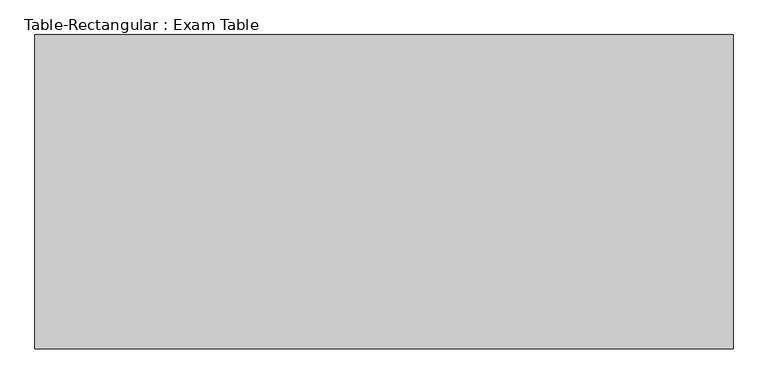
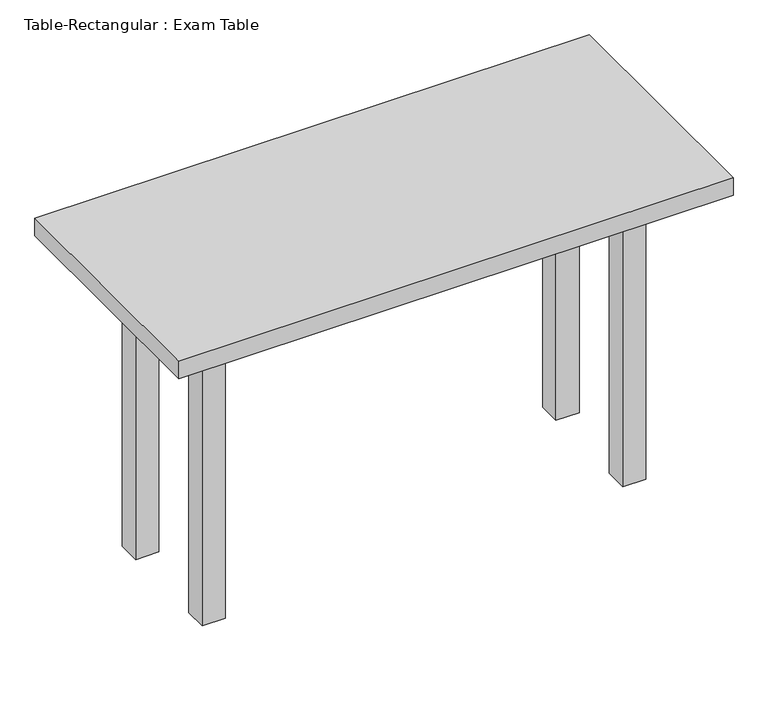
"""IFC4 building model written with IfcOpenShell, lengths in millimetres: furniture geometry, Table-Rectangular : Exam Table."""

from ifc_helpers import new_model, si_unit, frame, origin, origin_with_axes, place, context, project, spatial, polyline, outline, extrude, source, transform, mapped, element, save


def table_rectangular_exam_table_7d83067c(model_context):
    return source(origin(), model_context, "Body", "SweptSolid", [
        extrude(outline(polyline([(546.1, 152.4), (546.1, 127.0), (-546.1, 127.0), (-546.1, 152.4), (546.1, 152.4)])), frame((0.0, 0.0, 762.0), z_axis=(0.0, 0.0, 1.0), x_axis=(1.0, 0.0, 0.0)), (0.0, 0.0, 1.0), 101.6),
        extrude(outline(polyline([(546.1, -152.4), (-546.1, -152.4), (-546.1, -127.0), (546.1, -127.0), (546.1, -152.4)])), frame((0.0, 0.0, 762.0), z_axis=(0.0, 0.0, 1.0), x_axis=(1.0, 0.0, 0.0)), (0.0, 0.0, 1.0), 101.6),
        extrude(outline(polyline([(-558.8, -127.0), (-584.2, -127.0), (-584.2, 127.0), (-558.8, 127.0), (-558.8, -127.0)])), frame((0.0, 0.0, 762.0), z_axis=(0.0, 0.0, 1.0), x_axis=(1.0, 0.0, 0.0)), (0.0, 0.0, 1.0), 101.6),
        extrude(outline(polyline([(558.8, -127.0), (558.8, 127.0), (584.2, 127.0), (584.2, -127.0), (558.8, -127.0)])), frame((0.0, 0.0, 762.0), z_axis=(0.0, 0.0, 1.0), x_axis=(1.0, 0.0, 0.0)), (0.0, 0.0, 1.0), 101.6),
        extrude(outline(polyline([(762.0, 342.9), (762.0, -342.9), (-762.0, -342.9), (-762.0, 342.9), (762.0, 342.9)])), frame((0.0, 0.0, 863.6), z_axis=(0.0, 0.0, 1.0), x_axis=(1.0, 0.0, 0.0)), (0.0, 0.0, 1.0), 50.8),
        extrude(outline(polyline([(-546.1, 190.5), (-546.1, 127.0), (-609.6, 127.0), (-609.6, 190.5), (-546.1, 190.5)])), origin_with_axes(), (0.0, 0.0, 1.0), 863.6),
        extrude(outline(polyline([(546.1, 190.5), (609.6, 190.5), (609.6, 127.0), (546.1, 127.0), (546.1, 190.5)])), origin_with_axes(), (0.0, 0.0, 1.0), 863.6),
        extrude(outline(polyline([(-546.1, -190.5), (-609.6, -190.5), (-609.6, -127.0), (-546.1, -127.0), (-546.1, -190.5)])), origin_with_axes(), (0.0, 0.0, 1.0), 863.6),
        extrude(outline(polyline([(546.1, -190.5), (546.1, -127.0), (609.6, -127.0), (609.6, -190.5), (546.1, -190.5)])), origin_with_axes(), (0.0, 0.0, 1.0), 863.6),
    ])


if __name__ == "__main__":
    model = new_model("IFC4")
    model_context = context("Model", 3, world=origin())
    ifc_project = project(units=[si_unit("LENGTHUNIT", "METRE", prefix="MILLI")], contexts=[model_context])
    site = spatial("IfcSite", under=ifc_project)
    building = spatial("IfcBuilding", under=site)
    placement = place(None, origin())
    table_rectangular_exam_table_shape = table_rectangular_exam_table_7d83067c(model_context)
    element("IfcFurniture", 1, ObjectType="Table-Rectangular : Exam Table", at=placement, inside=building, context=model_context, shape_type="MappedRepresentation", body=[
        mapped(table_rectangular_exam_table_shape, transform((0.0, 0.0, 0.0), x_axis=(1.0, 0.0, 0.0), y_axis=(0.0, 1.0, 0.0), z_axis=(0.0, 0.0, 1.0))),
    ])
    save(model, "model.ifc")

# Revit data of these elements
# Type "Table-Rectangular : Exam Table"
#   Assembly Code = "E2020200"
#   Height = 3' - 0"
#   Length = 5' - 0"
#   Width = 2' - 3"
#   Base Material = Wood - Birch
#   Top Material = Wood - Birch
#   Default Elevation = 0
# Element 1 (IfcFurniture, "Table-Rectangular : Exam Table")
#   Materials on its faces: "Wood - Birch"
# Materials
#   "Wood - Birch": class "Unassigned", colour RGB 224 178 126, transparency 0
